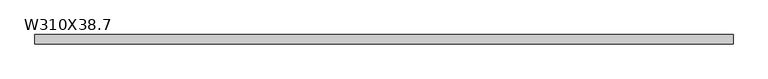
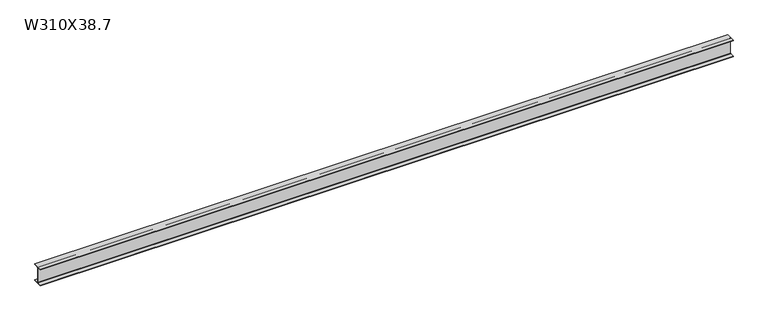
"""IFC4 building model written with IfcOpenShell, lengths in millimetres: beam geometry, M_W Shapes : W310X38.7."""

from ifc_helpers import new_model, si_unit, point, frame, frame_2d, origin, place, context, project, spatial, polyline, circle_curve, trimmed, segment, composite_curve, outline, extrude, source, transform, mapped, element, save


def w310x38_7_2c265120(model_context):
    return source(origin(), model_context, "Body", "SweptSolid", [
        extrude(outline(composite_curve([segment(polyline([(82.5, -145.35), (82.5, -155.0), (-82.5, -155.0), (-82.5, -145.35), (-10.57, -145.35)]), True, "CONTINUOUS"), segment(trimmed(circle_curve(frame_2d((-10.57, -137.7)), 7.65), [point((-10.57, -145.35))], [point((-2.92, -137.7))], True, "CARTESIAN"), True, "CONTINUOUS"), segment(polyline([(-2.92, -137.7), (-2.92, 137.7)]), True, "CONTINUOUS"), segment(trimmed(circle_curve(frame_2d((-10.57, 137.7)), 7.65), [point((-2.92, 137.7))], [point((-10.57, 145.35))], True, "CARTESIAN"), True, "CONTINUOUS"), segment(polyline([(-10.57, 145.35), (-82.5, 145.35), (-82.5, 155.0), (82.5, 155.0), (82.5, 145.35), (10.57, 145.35)]), True, "CONTINUOUS"), segment(trimmed(circle_curve(frame_2d((10.57, 137.7)), 7.65), [point((10.57, 145.35))], [point((2.92, 137.7))], True, "CARTESIAN"), True, "CONTINUOUS"), segment(polyline([(2.92, 137.7), (2.92, -137.7)]), True, "CONTINUOUS"), segment(trimmed(circle_curve(frame_2d((10.57, -137.7)), 7.65), [point((2.92, -137.7))], [point((10.57, -145.35))], True, "CARTESIAN"), True, "CONTINUOUS"), segment(polyline([(10.57, -145.35), (82.5, -145.35)]), True, "CONTINUOUS")], self_intersect=False)), frame((-6194.75, 0.0, 0.0), z_axis=(1.0, 0.0, 0.0), x_axis=(0.0, 1.0, 0.0)), (0.0, 0.0, 1.0), 12271.9),
    ])


if __name__ == "__main__":
    model = new_model("IFC4")
    model_context = context("Model", 3, world=origin())
    ifc_project = project(units=[si_unit("LENGTHUNIT", "METRE", prefix="MILLI")], contexts=[model_context])
    site = spatial("IfcSite", under=ifc_project)
    building = spatial("IfcBuilding", under=site)
    placement = place(None, origin())
    w310x38_7_shape = w310x38_7_2c265120(model_context)
    element("IfcBeam", 1, ObjectType="M_W Shapes : W310X38.7", at=placement, inside=building, context=model_context, shape_type="MappedRepresentation", body=[
        mapped(w310x38_7_shape, transform((0.0, 0.0, 0.0), x_axis=(1.0, 0.0, 0.0), y_axis=(0.0, 1.0, 0.0), z_axis=(0.0, 0.0, 1.0))),
    ])
    save(model, "model.ifc")

# Revit data of these elements
# Type "M_W Shapes : W310X38.7"
#   Section Name Key = "W12x26"
#   Width = 165 mm
#   Web Thickness = 5.84 mm
#   Web Fillet = 7.65 mm
#   Warping Constant = 163000 cm⁶
#   Torsional Moment of Inertia = 12.5 cm⁴
#   Section Area = 49.4 cm²
#   Plastic Modulus weak axis = 0.00473217 (stored number, unit not read)
#   Plastic Modulus strong axis = 0.0215419 (stored number, unit not read)
#   Perimeter = 1.25 m²/m
#   Nominal Weight = 379.516 N/m
#   Moment of Inertia weak axis = 720 cm⁴
#   Moment of Inertia strong axis = 8490 cm⁴
#   Height = 310 mm
#   Flange Thickness = 9.65 mm
#   Elastic Modulus weak axis = 0.00309003 (stored number, unit not read)
#   Elastic Modulus strong axis = 0.0193171 (stored number, unit not read)
#   Centroid Vertical = 155 mm
#   Centroid Horizontal = 82.5 mm
#   Length [instance default] = 1.5 m
#   Structural Material [instance default] = Steel, 45-345
#   Assembly Code = ""
# Element 1 (IfcBeam, "M_W Shapes : W310X38.7")
#   Materials on its faces: "Steel, 45-345"
# Materials
#   "Steel, 45-345": class "Metal", colour RGB 189 187 185, transparency 0, Description = "Steel 345 MPa", Cost = 0
